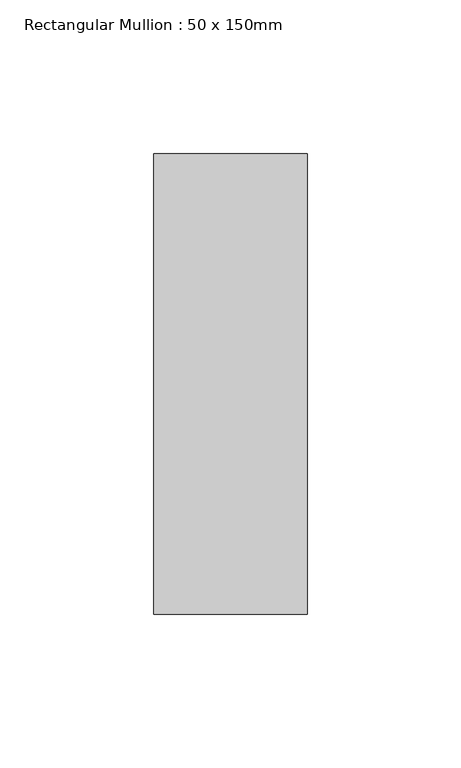
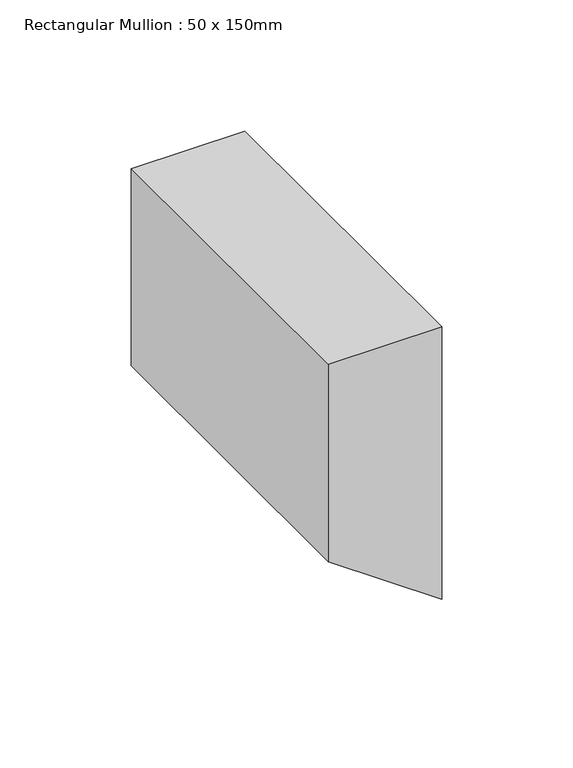
"""IFC4 building model written with IfcOpenShell, lengths in millimetres: member geometry, Rectangular Mullion : 50 x 150mm."""

from ifc_helpers import new_model, si_unit, frame, origin, place, context, project, spatial, polyline, outline, extrude, source, transform, mapped, element, save


def rectangular_mullion_50_x_150mm_a7d84edf(model_context):
    return source(origin(), model_context, "Body", "SweptSolid", [
        extrude(outline(polyline([(0.0, 25.0), (0.0, -25.0), (-91.6843741, -25.0), (-126.694751, 25.0), (0.0, 25.0)])), frame((0.0, -75.0, 0.0), z_axis=(0.0, 1.0, 0.0), x_axis=(0.0, 0.0, 1.0)), (0.0, 0.0, 1.0), 150.0),
    ])


if __name__ == "__main__":
    model = new_model("IFC4")
    model_context = context("Model", 3, world=origin())
    ifc_project = project(units=[si_unit("LENGTHUNIT", "METRE", prefix="MILLI")], contexts=[model_context])
    site = spatial("IfcSite", under=ifc_project)
    building = spatial("IfcBuilding", under=site)
    placement = place(None, origin())
    rectangular_mullion_50_x_150mm_shape = rectangular_mullion_50_x_150mm_a7d84edf(model_context)
    element("IfcMember", 1, ObjectType="Rectangular Mullion : 50 x 150mm", at=placement, inside=building, context=model_context, shape_type="MappedRepresentation", body=[
        mapped(rectangular_mullion_50_x_150mm_shape, transform((0.0, 0.0, 0.0), x_axis=(1.0, 0.0, 0.0), y_axis=(0.0, 1.0, 0.0), z_axis=(0.0, 0.0, 1.0))),
    ])
    save(model, "model.ifc")

# Revit data of these elements
# Type "Rectangular Mullion : 50 x 150mm"
#   built-in parameter 1007304 = 0.492126 (stored number, unit not read)
#   built-in parameter 1007301 = 0.082021 (stored number, unit not read)
#   built-in parameter 1007300 = 0.082021 (stored number, unit not read)
# Element 1 (IfcMember, "Rectangular Mullion : 50 x 150mm")
#   Materials on its faces: "Aluminium"
# Materials
#   "Aluminium": class "Metal", colour RGB 247 247 247, transparency 0, Description = "Aluminium 6061", Cost = 0
